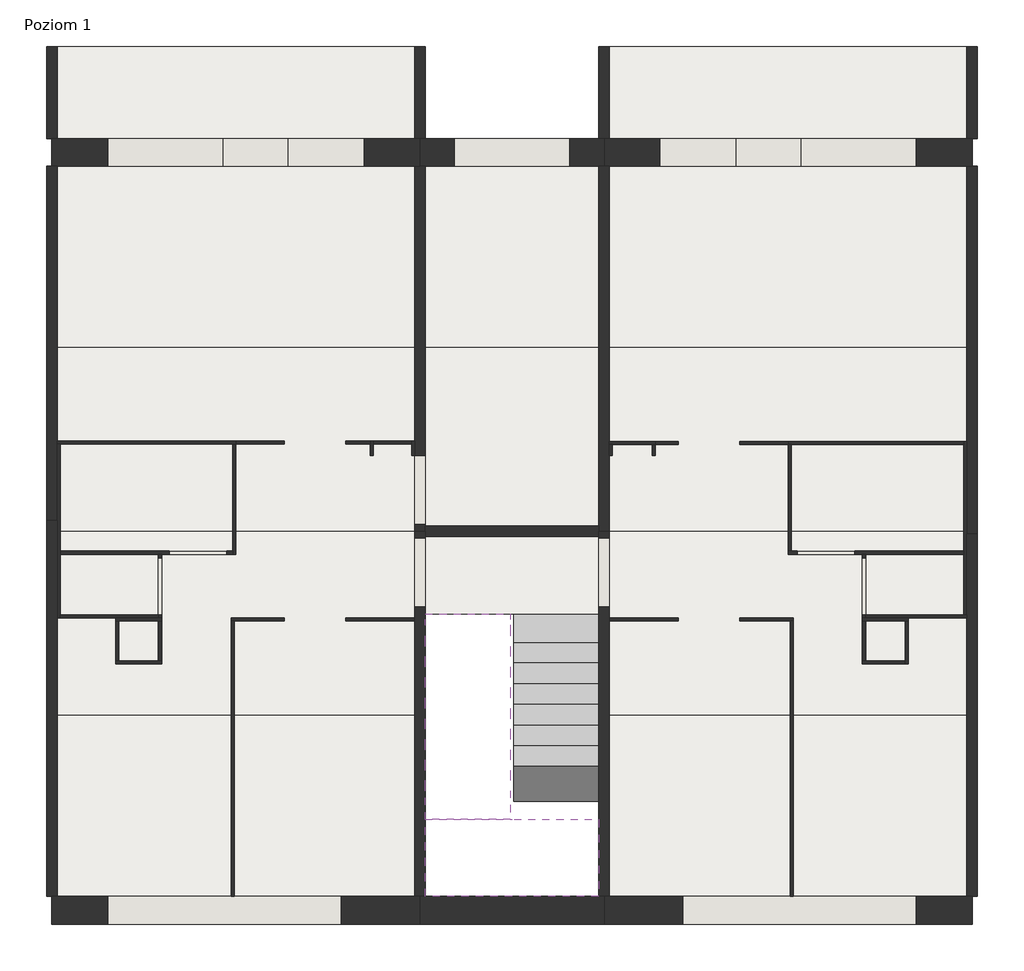
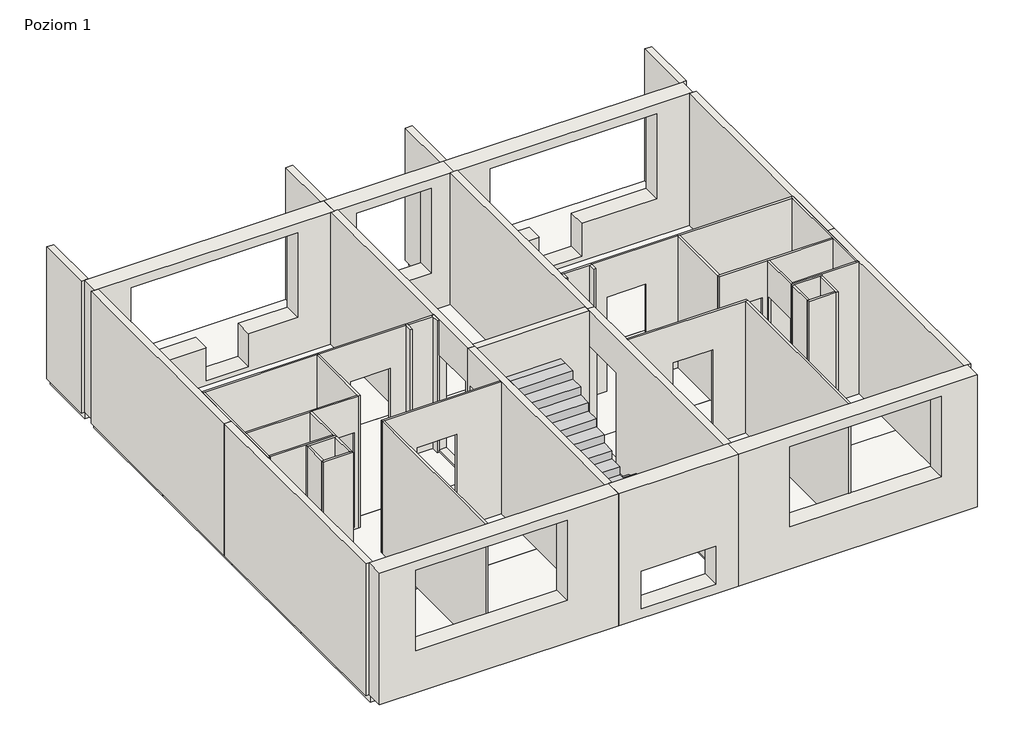
# One storey: 51 walls, 14 slabs, 2 proxies.
"""IFC4 building model written with IfcOpenShell, lengths in millimetres."""

import ifcopenshell
import ifcopenshell.guid

model = None  # the IFC model being written
_history = None  # IfcOwnerHistory: only IFC2X3 demands one
_inside = {}  # id of a spatial element -> (the spatial element, [elements in it])
_under = {}  # id of a project, library or spatial element -> (it, [spatial elements below it])
_declared = {}  # id of a project -> (the project, [libraries it declares])
_typed = {}  # id of a type object -> (the type object, [elements of that type])
_made_of = {}  # id of a material, layer set ... -> (it, [elements and type objects made of it])


def new_model(schema):
    """Start an empty IFC model of exactly this schema.

    Asked for "IFC4X3", IfcOpenShell would pick the latest addendum, in which some entities
    have other attributes; the version numbers below select the first issue.
    IFC2X3 requires an IfcOwnerHistory on every rooted entity: one is made here for all.
    """
    global model, _history
    if schema == "IFC4X3":
        model = ifcopenshell.file(schema_version=(4, 3, 0, 0))
    else:
        model = ifcopenshell.file(schema=schema)
    _inside.clear()
    _under.clear()
    _declared.clear()
    _typed.clear()
    _made_of.clear()
    _history = None
    if model.schema == "IFC2X3":
        org = make("IfcOrganization", Name="unknown")
        user = make(
            "IfcPersonAndOrganization",
            ThePerson=make("IfcPerson", FamilyName="unknown"),
            TheOrganization=org,
        )
        app = make(
            "IfcApplication",
            ApplicationDeveloper=org,
            Version="unknown",
            ApplicationFullName="unknown",
            ApplicationIdentifier="unknown",
        )
        _history = make(
            "IfcOwnerHistory",
            OwningUser=user,
            OwningApplication=app,
            ChangeAction="ADDED",
            CreationDate=0,
        )
    return model


def make(cls, **values):
    """One entity of the class cls with the attributes given. An attribute that is None is left unset."""
    return model.create_entity(
        cls, **{name: value for name, value in values.items() if value is not None}
    )


def rooted(cls, **values):
    """An entity with a GlobalId (a new one), such as an element, a storey or a relation."""
    return make(cls, GlobalId=ifcopenshell.guid.new(), OwnerHistory=_history, **values)


def si_unit(unit_type, name, prefix=None):
    """IfcSIUnit, for example si_unit("LENGTHUNIT", "METRE", prefix="MILLI")."""
    return make("IfcSIUnit", UnitType=unit_type, Prefix=prefix, Name=name)


def assignment(units):
    """IfcUnitAssignment: the units of a project."""
    return None if units is None else make("IfcUnitAssignment", Units=units)


def point(xyz):
    """IfcCartesianPoint."""
    return None if xyz is None else make("IfcCartesianPoint", Coordinates=xyz)


def direction(xyz):
    """IfcDirection."""
    return None if xyz is None else make("IfcDirection", DirectionRatios=xyz)


def frame(location, z_axis=None, x_axis=None):
    """IfcAxis2Placement3D, a coordinate frame: its origin and axes. An axis left out is left unset."""
    return make(
        "IfcAxis2Placement3D",
        Location=point(location),
        Axis=direction(z_axis),
        RefDirection=direction(x_axis),
    )


def origin():
    """The frame at (0, 0, 0) with its axes left unset."""
    return frame((0.0, 0.0, 0.0))


def origin_with_axes():
    """The frame at (0, 0, 0) with the z axis (0, 0, 1) and the x axis (1, 0, 0) written out."""
    return frame((0.0, 0.0, 0.0), z_axis=(0.0, 0.0, 1.0), x_axis=(1.0, 0.0, 0.0))


def place(relative_to, where):
    """IfcLocalPlacement: puts the frame where relative to a parent placement (None: the world)."""
    return make(
        "IfcLocalPlacement", PlacementRelTo=relative_to, RelativePlacement=where
    )


def context(
    kind, dimensions, precision=None, world=None, true_north=None, identifier=None
):
    """IfcGeometricRepresentationContext, for example the 3D "Model" context."""
    return make(
        "IfcGeometricRepresentationContext",
        ContextIdentifier=identifier,
        ContextType=kind,
        CoordinateSpaceDimension=dimensions,
        Precision=precision,
        WorldCoordinateSystem=world,
        TrueNorth=true_north,
    )


def project(units=None, contexts=None):
    """IfcProject with its units and contexts."""
    return rooted(
        "IfcProject",
        Name="project",
        RepresentationContexts=contexts,
        UnitsInContext=assignment(units),
    )


def spatial(cls, under=None, at=None, **own):
    """A site, building, storey or space (cls), placed at a placement, below another one or the project."""
    s = rooted(cls, ObjectPlacement=at, **own)
    if under is not None:
        _under.setdefault(under.id(), (under, []))[1].append(s)
    return s


def polyline(points):
    """IfcPolyline through the points."""
    return make("IfcPolyline", Points=[point(p) for p in points])


def outline(outer, holes=None, kind="AREA"):
    """IfcArbitraryClosedProfileDef: a profile drawn as a closed curve; with holes, ...WithVoids."""
    if holes is None:
        return make("IfcArbitraryClosedProfileDef", ProfileType=kind, OuterCurve=outer)
    return make(
        "IfcArbitraryProfileDefWithVoids",
        ProfileType=kind,
        OuterCurve=outer,
        InnerCurves=holes,
    )


def extrude(swept, where, along, depth):
    """IfcExtrudedAreaSolid: the profile swept, set in the frame where, extruded along a direction by depth."""
    return make(
        "IfcExtrudedAreaSolid",
        SweptArea=swept,
        Position=where,
        ExtrudedDirection=direction(along),
        Depth=depth,
    )


def faces_of(points, faces, orient=None, outer=None):
    """IfcFace entities. A face is a list of loops; a loop is a list of indices into points, from 0.

    orient and outer hold one flag for each loop. By default every Orientation is true, the
    first loop of a face is its IfcFaceOuterBound and the others are IfcFaceBound.
    """
    made = []
    for i, loops in enumerate(faces):
        bounds = []
        for j, loop in enumerate(loops):
            is_outer = j == 0 if outer is None else outer[i][j]
            bounds.append(
                make(
                    "IfcFaceOuterBound" if is_outer else "IfcFaceBound",
                    Bound=make("IfcPolyLoop", Polygon=[points[k] for k in loop]),
                    Orientation=True if orient is None else orient[i][j],
                )
            )
        made.append(make("IfcFace", Bounds=bounds))
    return made


def faceted_brep(points, faces, orient=None, outer=None, voids=None):
    """IfcFacetedBrep: a solid bounded by flat faces; with voids (closed shells), ...WithVoids."""
    shared = [point(p) for p in points]
    hull = make("IfcClosedShell", CfsFaces=faces_of(shared, faces, orient, outer))
    if voids is None:
        return make("IfcFacetedBrep", Outer=hull)
    return make(
        "IfcFacetedBrepWithVoids",
        Outer=hull,
        Voids=[
            make(cls, CfsFaces=faces_of(shared, fs, o, b)) for cls, fs, o, b in voids
        ],
    )


def shape(context_of_items, identifier, shape_type, items):
    """IfcShapeRepresentation: the items that make up one representation, for example the "Body"."""
    return make(
        "IfcShapeRepresentation",
        ContextOfItems=context_of_items,
        RepresentationIdentifier=identifier,
        RepresentationType=shape_type,
        Items=items,
    )


def source(mapping_origin, context_of_items, identifier, shape_type, items):
    """IfcRepresentationMap: a shape defined once, which mapped items show again and again."""
    return make(
        "IfcRepresentationMap",
        MappingOrigin=mapping_origin,
        MappedRepresentation=shape(context_of_items, identifier, shape_type, items),
    )


def transform(
    local_origin,
    x_axis=None,
    y_axis=None,
    z_axis=None,
    scale=None,
    scale2=None,
    scale3=None,
    uniform=True,
):
    """IfcCartesianTransformationOperator3D, or its non-uniform kind. x_axis, y_axis, z_axis: its Axis1, 2, 3."""
    if uniform:
        return make(
            "IfcCartesianTransformationOperator3D",
            Axis1=direction(x_axis),
            Axis2=direction(y_axis),
            LocalOrigin=point(local_origin),
            Scale=scale,
            Axis3=direction(z_axis),
        )
    return make(
        "IfcCartesianTransformationOperator3DnonUniform",
        Axis1=direction(x_axis),
        Axis2=direction(y_axis),
        LocalOrigin=point(local_origin),
        Scale=scale,
        Axis3=direction(z_axis),
        Scale2=scale2,
        Scale3=scale3,
    )


def mapped(mapping_source, mapping_target):
    """IfcMappedItem: shows the shape of a source again, moved by a transform."""
    return make(
        "IfcMappedItem", MappingSource=mapping_source, MappingTarget=mapping_target
    )


def made_of(thing, what):
    """Note that an element or type object is made of a material, layer set ...; save() writes the relation."""
    if what is not None:
        _made_of.setdefault(what.id(), (what, []))[1].append(thing)
    return thing


def element(
    cls,
    number,
    at=None,
    inside=None,
    cuts=None,
    type_object=None,
    material=None,
    context=None,
    identifier="Body",
    shape_type=None,
    held_by="IfcProductDefinitionShape",
    body=None,
    shapes=None,
    **own,
):
    """One element of the class cls, such as IfcWall. Its Tag is "e" and its number.

    at: its placement. inside: the storey or other place that contains it. cuts: it is an
    opening in that element (IfcRelVoidsElement). A single representation is given by context,
    identifier, shape_type and body (its items); several are given by shapes. held_by: the class
    of the entity that holds the representations. save() writes the other relations.
    """
    e = rooted(cls, Tag="e%d" % number, ObjectPlacement=at, **own)
    if body is not None:
        shapes = [shape(context, identifier, shape_type, body)]
    if shapes is not None:
        e.Representation = make(held_by, Representations=shapes)
    if inside is not None:
        _inside.setdefault(inside.id(), (inside, []))[1].append(e)
    if cuts is not None:
        rooted(
            "IfcRelVoidsElement", RelatingBuildingElement=cuts, RelatedOpeningElement=e
        )
    if type_object is not None:
        _typed.setdefault(type_object.id(), (type_object, []))[1].append(e)
    return made_of(e, material)


def aggregate(whole, parts):
    """IfcRelAggregates: a whole, such as a stair, and the parts it consists of."""
    return rooted("IfcRelAggregates", RelatingObject=whole, RelatedObjects=parts)


def save(model, path):
    """Write the relations noted so far, then the file.

    IfcRelAggregates (storeys below a building ...), IfcRelContainedInSpatialStructure (elements
    in a storey), IfcRelDefinesByType, IfcRelAssociatesMaterial and IfcRelDeclares: one each for
    every whole, place, type object, material and project.
    """
    for whole, parts in _under.values():
        aggregate(whole, parts)
    for where, things in _inside.values():
        rooted(
            "IfcRelContainedInSpatialStructure",
            RelatedElements=things,
            RelatingStructure=where,
        )
    for kind, things in _typed.values():
        rooted("IfcRelDefinesByType", RelatedObjects=things, RelatingType=kind)
    for what, things in _made_of.values():
        rooted("IfcRelAssociatesMaterial", RelatedObjects=things, RelatingMaterial=what)
    for by, libraries in _declared.values():
        rooted("IfcRelDeclares", RelatingContext=by, RelatedDefinitions=libraries)
    model.write(path)


def generic_models_1_generic_models_1_c3b3df0b(model_context):
    return source(origin(), model_context, "Body", "SweptSolid", [
        extrude(outline(polyline([(23365.484552, 1575.0), (23630.484552, 1575.0), (23630.484552, 1750.0), (23900.484552, 1750.0), (23900.484552, 1925.0), (24170.484552, 1925.0), (24170.484552, 2100.0), (24440.484552, 2100.0), (24440.484552, 2273.0), (24710.484552, 2273.0), (24710.484552, 2450.0), (24980.484552, 2450.0), (24980.484552, 2625.0), (25250.484552, 2625.0), (25250.484552, 2800.0), (25520.484552, 2800.0), (25670.484552, 2800.0), (25670.484552, 2660.0), (25525.484552, 2660.0), (23365.484552, 1260.0), (22990.484552, 1260.0), (22990.484552, 1400.0), (23365.484552, 1400.0), (23365.484552, 1575.0)])), frame((81451.2978475, 0.0, 0.0), z_axis=(1.0, 0.0, 0.0), x_axis=(0.0, 1.0, 0.0)), (0.0, 0.0, 1.0), 1105.7161874),
    ])


def generic_models_3_generic_models_1_35d45e08(model_context):
    return source(origin(), model_context, "Body", "SweptSolid", [
        extrude(outline(polyline([(25295.484552, 175.0), (25295.484552, 0.0), (25670.484552, 0.0), (25670.484552, -140.0), (25295.484552, -140.0), (23135.484552, 1260.0), (22990.484552, 1260.0), (22990.484552, 1400.0), (23140.484552, 1400.0), (23410.484552, 1400.0), (23410.484552, 1225.0), (23680.484552, 1225.0), (23680.484552, 1050.0), (23950.484552, 1050.0), (23950.484552, 873.0), (24220.484552, 873.0), (24220.484552, 700.0), (24490.484552, 700.0), (24490.484552, 525.0), (24760.484552, 525.0), (24760.484552, 350.0), (25030.484552, 350.0), (25030.484552, 175.0), (25295.484552, 175.0)])), frame((82605.5816601, 0.0, 0.0), z_axis=(1.0, 0.0, 0.0), x_axis=(0.0, 1.0, 0.0)), (0.0, 0.0, 1.0), 1105.7161874),
    ])


model = new_model("IFC4")

# Units and contexts
model_context = context("Model", 3, world=origin())
ifc_project = project(units=[si_unit("LENGTHUNIT", "METRE", prefix="MILLI")], contexts=[model_context])

# Site, building, storey
site = spatial("IfcSite", under=ifc_project)
building = spatial("IfcBuilding", under=site)
storey = spatial("IfcBuildingStorey", under=building, Name="Poziom 1", Elevation=0.0)

# Proxies
placement = place(None, origin())
generic_models_1_generic_models_1_shape = generic_models_1_generic_models_1_c3b3df0b(model_context)
element("IfcBuildingElementProxy", 1, Name="Generic Models 1 : Generic Models 1", ObjectType="Generic Models 1 : Generic Models 1", at=placement, inside=storey, context=model_context, shape_type="MappedRepresentation", body=[
    mapped(generic_models_1_generic_models_1_shape, transform((0.0, 0.0, 0.0), x_axis=(1.0, 0.0, 0.0), y_axis=(0.0, 1.0, 0.0), z_axis=(0.0, 0.0, 1.0))),
])
generic_models_3_generic_models_1_shape = generic_models_3_generic_models_1_35d45e08(model_context)
element("IfcBuildingElementProxy", 2, Name="Generic Models 3 : Generic Models 1", ObjectType="Generic Models 3 : Generic Models 1", at=placement, inside=storey, context=model_context, shape_type="MappedRepresentation", body=[
    mapped(generic_models_3_generic_models_1_shape, transform((0.0, 0.0, 0.0), x_axis=(1.0, 0.0, 0.0), y_axis=(0.0, 1.0, 0.0), z_axis=(0.0, 0.0, 1.0))),
])

# Slabs
element("IfcSlab", 3, ObjectType="Prefab_slab", at=placement, inside=storey, context=model_context, shape_type="SweptSolid", body=[
    extrude(outline(polyline([(81381.2978475, 24350.484552), (81381.2978475, 21950.484552), (76581.2978475, 21950.484552), (76581.2978475, 24350.484552), (81381.2978475, 24350.484552)])), frame((0.0, 0.0, -140.0), z_axis=(0.0, 0.0, 1.0), x_axis=(1.0, 0.0, 0.0)), (0.0, 0.0, 1.0), 140.0),
])
element("IfcSlab", 4, ObjectType="Prefab_slab", at=placement, inside=storey, context=model_context, shape_type="SweptSolid", body=[
    extrude(outline(polyline([(81381.2978475, 26750.484552), (81381.2978475, 24350.484552), (76581.2978475, 24350.484552), (76581.2978475, 26750.484552), (81381.2978475, 26750.484552)])), frame((0.0, 0.0, -140.0), z_axis=(0.0, 0.0, 1.0), x_axis=(1.0, 0.0, 0.0)), (0.0, 0.0, 1.0), 140.0),
])
element("IfcSlab", 5, ObjectType="Prefab_slab", at=placement, inside=storey, context=model_context, shape_type="SweptSolid", body=[
    extrude(outline(polyline([(81381.2978475, 29150.484552), (81381.2978475, 26750.484552), (76581.2978475, 26750.484552), (76581.2978475, 29150.484552), (81381.2978475, 29150.484552)])), frame((0.0, 0.0, -140.0), z_axis=(0.0, 0.0, 1.0), x_axis=(1.0, 0.0, 0.0)), (0.0, 0.0, 1.0), 140.0),
])
element("IfcSlab", 6, ObjectType="Prefab_slab", at=placement, inside=storey, context=model_context, shape_type="SweptSolid", body=[
    extrude(outline(polyline([(81381.2978475, 31550.484552), (81381.2978475, 29150.484552), (76581.2978475, 29150.484552), (76581.2978475, 31550.484552), (81381.2978475, 31550.484552)])), frame((0.0, 0.0, -140.0), z_axis=(0.0, 0.0, 1.0), x_axis=(1.0, 0.0, 0.0)), (0.0, 0.0, 1.0), 140.0),
])
element("IfcSlab", 7, ObjectType="Prefab_slab", at=placement, inside=storey, context=model_context, shape_type="SweptSolid", body=[
    extrude(outline(polyline([(88581.2978475, 24350.484552), (88581.2978475, 21950.484552), (83781.2978475, 21950.484552), (83781.2978475, 24350.484552), (88581.2978475, 24350.484552)])), frame((0.0, 0.0, -140.0), z_axis=(0.0, 0.0, 1.0), x_axis=(1.0, 0.0, 0.0)), (0.0, 0.0, 1.0), 140.0),
])
element("IfcSlab", 8, ObjectType="Prefab_slab", at=placement, inside=storey, context=model_context, shape_type="SweptSolid", body=[
    extrude(outline(polyline([(88581.2978475, 26750.484552), (88581.2978475, 24350.484552), (83781.2978475, 24350.484552), (83781.2978475, 26750.484552), (88581.2978475, 26750.484552)])), frame((0.0, 0.0, -140.0), z_axis=(0.0, 0.0, 1.0), x_axis=(1.0, 0.0, 0.0)), (0.0, 0.0, 1.0), 140.0),
])
element("IfcSlab", 9, ObjectType="Prefab_slab", at=placement, inside=storey, context=model_context, shape_type="SweptSolid", body=[
    extrude(outline(polyline([(88581.2978475, 29150.484552), (88581.2978475, 26750.484552), (83781.2978475, 26750.484552), (83781.2978475, 29150.484552), (88581.2978475, 29150.484552)])), frame((0.0, 0.0, -140.0), z_axis=(0.0, 0.0, 1.0), x_axis=(1.0, 0.0, 0.0)), (0.0, 0.0, 1.0), 140.0),
])
element("IfcSlab", 10, ObjectType="Prefab_slab", at=placement, inside=storey, context=model_context, shape_type="SweptSolid", body=[
    extrude(outline(polyline([(88581.2978475, 31550.484552), (88581.2978475, 29150.484552), (83781.2978475, 29150.484552), (83781.2978475, 31550.484552), (88581.2978475, 31550.484552)])), frame((0.0, 0.0, -140.0), z_axis=(0.0, 0.0, 1.0), x_axis=(1.0, 0.0, 0.0)), (0.0, 0.0, 1.0), 140.0),
])
element("IfcSlab", 11, ObjectType="Prefab_slab", at=placement, inside=storey, context=model_context, shape_type="SweptSolid", body=[
    extrude(outline(polyline([(83781.2978475, 31550.484552), (83781.2978475, 29150.484552), (81451.2978475, 29150.484552), (81451.2978475, 31550.484552), (83781.2978475, 31550.484552)])), frame((0.0, 0.0, -140.0), z_axis=(0.0, 0.0, 1.0), x_axis=(1.0, 0.0, 0.0)), (0.0, 0.0, 1.0), 140.0),
])
element("IfcSlab", 12, ObjectType="Prefab_slab", at=placement, inside=storey, context=model_context, shape_type="SweptSolid", body=[
    extrude(outline(polyline([(83781.2978475, 29150.484552), (83781.2978475, 26750.484552), (81451.2978475, 26750.484552), (81451.2978475, 29150.484552), (83781.2978475, 29150.484552)])), frame((0.0, 0.0, -140.0), z_axis=(0.0, 0.0, 1.0), x_axis=(1.0, 0.0, 0.0)), (0.0, 0.0, 1.0), 140.0),
])
element("IfcSlab", 13, ObjectType="Prefab_slab", at=placement, inside=storey, context=model_context, shape_type="SweptSolid", body=[
    extrude(outline(polyline([(83781.2978475, 26750.484552), (83781.2978475, 25670.484552), (81451.2978475, 25670.484552), (81451.2978475, 26750.484552), (83781.2978475, 26750.484552)])), frame((0.0, 0.0, -140.0), z_axis=(0.0, 0.0, 1.0), x_axis=(1.0, 0.0, 0.0)), (0.0, 0.0, 1.0), 140.0),
])
element("IfcSlab", 14, ObjectType="Prefab_slab", at=placement, inside=storey, context=model_context, shape_type="SweptSolid", body=[
    extrude(outline(polyline([(83711.2978475, 22990.484552), (83711.2978475, 21985.484552), (81451.2978475, 21985.484552), (81451.2978475, 22990.484552), (82558.3014634, 22990.484552), (82611.2978475, 22990.484552), (83711.2978475, 22990.484552)])), frame((0.0, 0.0, 1260.0), z_axis=(0.0, 0.0, 1.0), x_axis=(1.0, 0.0, 0.0)), (0.0, 0.0, 1.0), 140.0),
])
element("IfcSlab", 15, ObjectType="Prefab_slab 2", at=placement, inside=storey, context=model_context, shape_type="SweptSolid", body=[
    extrude(outline(polyline([(81381.2978475, 33075.484552), (81381.2978475, 31875.484552), (76581.2978475, 31875.484552), (76581.2978475, 33075.484552), (81381.2978475, 33075.484552)])), frame((0.0, 0.0, -140.0), z_axis=(0.0, 0.0, 1.0), x_axis=(1.0, 0.0, 0.0)), (0.0, 0.0, 1.0), 140.0),
])
element("IfcSlab", 16, ObjectType="Prefab_slab 2", at=placement, inside=storey, context=model_context, shape_type="SweptSolid", body=[
    extrude(outline(polyline([(88581.2978475, 33075.484552), (88581.2978475, 31875.484552), (83781.2978475, 31875.484552), (83781.2978475, 33075.484552), (88581.2978475, 33075.484552)])), frame((0.0, 0.0, -140.0), z_axis=(0.0, 0.0, 1.0), x_axis=(1.0, 0.0, 0.0)), (0.0, 0.0, 1.0), 140.0),
])

# Walls
element("IfcWall", 17, ObjectType="Prefab_ext_wall", at=placement, inside=storey, context=model_context, shape_type="SweptSolid", body=[
    extrude(outline(polyline([(0.0, 76581.2978475), (0.0, 81381.2978475), (2800.0, 81381.2978475), (2800.0, 76581.2978475), (0.0, 76581.2978475)]), holes=[polyline([(2600.0, 77311.2978475), (2600.0, 80651.2978475), (800.0, 80651.2978475), (800.0, 79661.2978475), (100.0, 79661.2978475), (100.0, 78811.2978475), (800.0, 78811.2978475), (800.0, 77311.2978475), (2600.0, 77311.2978475)])]), frame((0.0, 31515.484552, 0.0), z_axis=(0.0, 1.0, 0.0), x_axis=(0.0, 0.0, 1.0)), (0.0, 0.0, 1.0), 360.0),
])
element("IfcWall", 18, ObjectType="Prefab_ext_wall", at=placement, inside=storey, context=model_context, shape_type="SweptSolid", body=[
    extrude(outline(polyline([(0.0, 81381.2978475), (0.0, 83781.2978475), (2800.0, 83781.2978475), (2800.0, 81381.2978475), (0.0, 81381.2978475)]), holes=[polyline([(800.0, 83331.2978475), (800.0, 81831.2978475), (2600.0, 81831.2978475), (2600.0, 83331.2978475), (800.0, 83331.2978475)])]), frame((0.0, 31515.484552, 0.0), z_axis=(0.0, 1.0, 0.0), x_axis=(0.0, 0.0, 1.0)), (0.0, 0.0, 1.0), 360.0),
])
element("IfcWall", 19, ObjectType="Prefab_ext_wall", at=placement, inside=storey, context=model_context, shape_type="SweptSolid", body=[
    extrude(outline(polyline([(0.0, 83781.2978475), (0.0, 88581.2978475), (2800.0, 88581.2978475), (2800.0, 83781.2978475), (0.0, 83781.2978475)]), holes=[polyline([(800.0, 84511.2978475), (2600.0, 84511.2978475), (2600.0, 87851.2978475), (800.0, 87851.2978475), (800.0, 86351.2978475), (100.0, 86351.2978475), (100.0, 85501.2978475), (800.0, 85501.2978475), (800.0, 84511.2978475)])]), frame((0.0, 31515.484552, 0.0), z_axis=(0.0, 1.0, 0.0), x_axis=(0.0, 0.0, 1.0)), (0.0, 0.0, 1.0), 360.0),
])
element("IfcWall", 20, ObjectType="Prefab_ext_wall", at=placement, inside=storey, context=model_context, shape_type="SweptSolid", body=[
    extrude(outline(polyline([(0.0, 76581.2978475), (0.0, 81381.2978475), (2800.0, 81381.2978475), (2800.0, 76581.2978475), (0.0, 76581.2978475)]), holes=[polyline([(2600.0, 77311.2978475), (2600.0, 80351.2978475), (900.0, 80351.2978475), (900.0, 77311.2978475), (2600.0, 77311.2978475)])]), frame((0.0, 21625.484552, 0.0), z_axis=(0.0, 1.0, 0.0), x_axis=(0.0, 0.0, 1.0)), (0.0, 0.0, 1.0), 360.0),
])
element("IfcWall", 21, ObjectType="Prefab_ext_wall", at=placement, inside=storey, context=model_context, shape_type="SweptSolid", body=[
    extrude(outline(polyline([(0.0, 81381.2978475), (0.0, 83781.2978475), (2800.0, 83781.2978475), (2800.0, 81381.2978475), (0.0, 81381.2978475)]), holes=[polyline([(1000.0, 83331.2978475), (200.0, 83331.2978475), (200.0, 81831.2978475), (1000.0, 81831.2978475), (1000.0, 83331.2978475)])]), frame((0.0, 21625.484552, 0.0), z_axis=(0.0, 1.0, 0.0), x_axis=(0.0, 0.0, 1.0)), (0.0, 0.0, 1.0), 360.0),
])
element("IfcWall", 22, ObjectType="Prefab_ext_wall", at=placement, inside=storey, context=model_context, shape_type="SweptSolid", body=[
    extrude(outline(polyline([(0.0, 83781.2978475), (0.0, 88581.2978475), (2800.0, 88581.2978475), (2800.0, 83781.2978475), (0.0, 83781.2978475)]), holes=[polyline([(900.0, 87851.2978475), (900.0, 84811.2978475), (2600.0, 84811.2978475), (2600.0, 87851.2978475), (900.0, 87851.2978475)])]), frame((0.0, 21625.484552, 0.0), z_axis=(0.0, 1.0, 0.0), x_axis=(0.0, 0.0, 1.0)), (0.0, 0.0, 1.0), 360.0),
])
element("IfcWall", 23, ObjectType="Prefab_int_wall", at=placement, inside=storey, context=model_context, shape_type="Brep", body=[
    faceted_brep([(76651.2978475, 27890.484552, 0.0), (76691.2978475, 27890.484552, 0.0), (78941.2978475, 27890.484552, 0.0), (78981.2978475, 27890.484552, 0.0), (78981.2978475, 27890.484552, 2800.0), (78941.2978475, 27890.484552, 2800.0), (76691.2978475, 27890.484552, 2800.0), (76651.2978475, 27890.484552, 2800.0), (76651.2978475, 27930.484552, 0.0), (76651.2978475, 27930.484552, 2800.0), (78981.2978475, 27930.484552, 2800.0), (78981.2978475, 27930.484552, 0.0)], [[[0, 1, 2, 3, 4, 5, 6, 7]], [[8, 9, 10, 11]], [[3, 2, 1, 0, 8, 11]], [[4, 3, 11, 10]], [[7, 6, 5, 4, 10, 9]], [[0, 7, 9, 8]]]),
])
element("IfcWall", 24, ObjectType="Prefab_int_wall", at=placement, inside=storey, context=model_context, shape_type="Brep", body=[
    faceted_brep([(78921.2978475, 25580.484552, 0.0), (78961.2978475, 25580.484552, 0.0), (79611.2978475, 25580.484552, 0.0), (79611.2978475, 25580.484552, 2000.0), (80411.2978475, 25580.484552, 2000.0), (80411.2978475, 25580.484552, 0.0), (81311.2978475, 25580.484552, 0.0), (81311.2978475, 25580.484552, 2800.0), (78961.2978475, 25580.484552, 2800.0), (78921.2978475, 25580.484552, 2800.0), (78921.2978475, 25620.484552, 0.0), (78921.2978475, 25620.484552, 2800.0), (81311.2978475, 25620.484552, 2800.0), (81311.2978475, 25620.484552, 0.0), (80411.2978475, 25620.484552, 0.0), (80411.2978475, 25620.484552, 2000.0), (79611.2978475, 25620.484552, 2000.0), (79611.2978475, 25620.484552, 0.0)], [[[0, 1, 2, 3, 4, 5, 6, 7, 8, 9]], [[10, 11, 12, 13, 14, 15, 16, 17]], [[6, 5, 14, 13]], [[7, 6, 13, 12]], [[9, 8, 7, 12, 11]], [[2, 1, 0, 10, 17]], [[3, 2, 17, 16]], [[4, 3, 16, 15]], [[5, 4, 15, 14]], [[0, 9, 11, 10]]]),
])
element("IfcWall", 25, ObjectType="Prefab_int_wall", at=placement, inside=storey, context=model_context, shape_type="SweptSolid", body=[
    extrude(outline(polyline([(78921.2978475, 21985.484552), (78921.2978475, 25580.484552), (78961.2978475, 25580.484552), (78961.2978475, 21985.484552), (78921.2978475, 21985.484552)])), origin_with_axes(), (0.0, 0.0, 1.0), 2800.0),
])
element("IfcWall", 26, ObjectType="Prefab_int_wall", at=placement, inside=storey, context=model_context, shape_type="Brep", body=[
    faceted_brep([(83851.2978475, 25580.484552, 0.0), (84751.2978475, 25580.484552, 0.0), (84751.2978475, 25580.484552, 2000.0), (85551.2978475, 25580.484552, 2000.0), (85551.2978475, 25580.484552, 0.0), (86211.2978475, 25580.484552, 0.0), (86251.2978475, 25580.484552, 0.0), (86251.2978475, 25580.484552, 2800.0), (86211.2978475, 25580.484552, 2800.0), (83851.2978475, 25580.484552, 2800.0), (83851.2978475, 25620.484552, 0.0), (83851.2978475, 25620.484552, 2800.0), (86251.2978475, 25620.484552, 2800.0), (86251.2978475, 25620.484552, 0.0), (85551.2978475, 25620.484552, 0.0), (85551.2978475, 25620.484552, 2000.0), (84751.2978475, 25620.484552, 2000.0), (84751.2978475, 25620.484552, 0.0)], [[[0, 1, 2, 3, 4, 5, 6, 7, 8, 9]], [[10, 11, 12, 13, 14, 15, 16, 17]], [[7, 6, 13, 12]], [[0, 9, 11, 10]], [[6, 5, 4, 14, 13]], [[9, 8, 7, 12, 11]], [[1, 0, 10, 17]], [[2, 1, 17, 16]], [[3, 2, 16, 15]], [[4, 3, 15, 14]]]),
])
element("IfcWall", 27, ObjectType="Prefab_int_wall", at=placement, inside=storey, context=model_context, shape_type="SweptSolid", body=[
    extrude(outline(polyline([(86211.2978475, 21985.484552), (86211.2978475, 25580.484552), (86251.2978475, 25580.484552), (86251.2978475, 21985.484552), (86211.2978475, 21985.484552)])), origin_with_axes(), (0.0, 0.0, 1.0), 2800.0),
])
element("IfcWall", 28, ObjectType="Prefab_int_wall", at=placement, inside=storey, context=model_context, shape_type="Brep", body=[
    faceted_brep([(87151.2978475, 25580.484552, 0.0), (87191.2978475, 25580.484552, 0.0), (87711.2978475, 25580.484552, 0.0), (87751.2978475, 25580.484552, 0.0), (87751.2978475, 25580.484552, 2800.0), (87711.2978475, 25580.484552, 2800.0), (87191.2978475, 25580.484552, 2800.0), (87151.2978475, 25580.484552, 2800.0), (87151.2978475, 25620.484552, 0.0), (87151.2978475, 25620.484552, 2800.0), (87751.2978475, 25620.484552, 2800.0), (87751.2978475, 25620.484552, 0.0)], [[[0, 1, 2, 3, 4, 5, 6, 7]], [[8, 9, 10, 11]], [[3, 2, 1, 0, 8, 11]], [[7, 6, 5, 4, 10, 9]], [[4, 3, 11, 10]], [[0, 7, 9, 8]]]),
])
element("IfcWall", 29, ObjectType="Prefab_int_wall", at=placement, inside=storey, context=model_context, shape_type="Brep", body=[
    faceted_brep([(87711.2978475, 25580.484552, 0.0), (87711.2978475, 25060.484552, 0.0), (87711.2978475, 25020.484552, 0.0), (87711.2978475, 25020.484552, 2800.0), (87711.2978475, 25060.484552, 2800.0), (87711.2978475, 25580.484552, 2800.0), (87751.2978475, 25580.484552, 0.0), (87751.2978475, 25580.484552, 2800.0), (87751.2978475, 25020.484552, 2800.0), (87751.2978475, 25020.484552, 0.0)], [[[0, 1, 2, 3, 4, 5]], [[6, 7, 8, 9]], [[2, 1, 0, 6, 9]], [[5, 4, 3, 8, 7]], [[0, 5, 7, 6]], [[3, 2, 9, 8]]]),
])
element("IfcWall", 30, ObjectType="Prefab_int_wall", at=placement, inside=storey, context=model_context, shape_type="Brep", body=[
    faceted_brep([(87711.2978475, 25060.484552, 0.0), (87191.2978475, 25060.484552, 0.0), (87151.2978475, 25060.484552, 0.0), (87151.2978475, 25060.484552, 2800.0), (87191.2978475, 25060.484552, 2800.0), (87711.2978475, 25060.484552, 2800.0), (87711.2978475, 25020.484552, 0.0), (87711.2978475, 25020.484552, 2800.0), (87151.2978475, 25020.484552, 2800.0), (87151.2978475, 25020.484552, 0.0)], [[[0, 1, 2, 3, 4, 5]], [[6, 7, 8, 9]], [[2, 1, 0, 6, 9]], [[5, 4, 3, 8, 7]], [[0, 5, 7, 6]], [[3, 2, 9, 8]]]),
])
element("IfcWall", 31, ObjectType="Prefab_int_wall", at=placement, inside=storey, context=model_context, shape_type="Brep", body=[
    faceted_brep([(87191.2978475, 25620.484552, 0.0), (87191.2978475, 25660.484552, 0.0), (87191.2978475, 26450.484552, 0.0), (87191.2978475, 26450.484552, 2800.0), (87191.2978475, 25660.484552, 2800.0), (87191.2978475, 25620.484552, 2800.0), (87191.2978475, 26400.484552, 2050.0), (87191.2978475, 26400.484552, 50.0), (87191.2978475, 25660.484552, 50.0), (87191.2978475, 25660.484552, 2050.0), (87151.2978475, 25620.484552, 0.0), (87151.2978475, 25620.484552, 2800.0), (87151.2978475, 26450.484552, 2800.0), (87151.2978475, 26450.484552, 0.0), (87151.2978475, 26400.484552, 2050.0), (87151.2978475, 25660.484552, 2050.0), (87151.2978475, 25660.484552, 50.0), (87151.2978475, 26400.484552, 50.0)], [[[0, 1, 2, 3, 4, 5], [6, 7, 8, 9]], [[10, 11, 12, 13], [14, 15, 16, 17]], [[3, 2, 13, 12]], [[2, 1, 0, 10, 13]], [[5, 4, 3, 12, 11]], [[0, 5, 11, 10]], [[7, 6, 14, 17]], [[8, 7, 17, 16]], [[6, 9, 15, 14]], [[9, 8, 16, 15]]]),
])
element("IfcWall", 32, ObjectType="Prefab_int_wall", at=placement, inside=storey, context=model_context, shape_type="Brep", body=[
    faceted_brep([(77411.2978475, 25580.484552, 0.0), (77451.2978475, 25580.484552, 0.0), (77971.2978475, 25580.484552, 0.0), (78011.2978475, 25580.484552, 0.0), (78011.2978475, 25580.484552, 2800.0), (77971.2978475, 25580.484552, 2800.0), (77451.2978475, 25580.484552, 2800.0), (77411.2978475, 25580.484552, 2800.0), (77411.2978475, 25620.484552, 0.0), (77411.2978475, 25620.484552, 2800.0), (78011.2978475, 25620.484552, 2800.0), (78011.2978475, 25620.484552, 0.0)], [[[0, 1, 2, 3, 4, 5, 6, 7]], [[8, 9, 10, 11]], [[3, 2, 1, 0, 8, 11]], [[7, 6, 5, 4, 10, 9]], [[0, 7, 9, 8]], [[4, 3, 11, 10]]]),
])
element("IfcWall", 33, ObjectType="Prefab_int_wall", at=placement, inside=storey, context=model_context, shape_type="Brep", body=[
    faceted_brep([(77971.2978475, 26450.484552, 0.0), (77971.2978475, 25660.484552, 0.0), (77971.2978475, 25620.484552, 0.0), (77971.2978475, 25620.484552, 2800.0), (77971.2978475, 25660.484552, 2800.0), (77971.2978475, 26450.484552, 2800.0), (77971.2978475, 25660.484552, 50.0), (77971.2978475, 26400.484552, 50.0), (77971.2978475, 26400.484552, 2050.0), (77971.2978475, 25660.484552, 2050.0), (78011.2978475, 26450.484552, 0.0), (78011.2978475, 26450.484552, 2800.0), (78011.2978475, 25620.484552, 2800.0), (78011.2978475, 25620.484552, 0.0), (78011.2978475, 25660.484552, 50.0), (78011.2978475, 25660.484552, 2050.0), (78011.2978475, 26400.484552, 2050.0), (78011.2978475, 26400.484552, 50.0)], [[[0, 1, 2, 3, 4, 5], [6, 7, 8, 9]], [[10, 11, 12, 13], [14, 15, 16, 17]], [[0, 5, 11, 10]], [[2, 1, 0, 10, 13]], [[3, 2, 13, 12]], [[5, 4, 3, 12, 11]], [[7, 6, 14, 17]], [[8, 7, 17, 16]], [[9, 8, 16, 15]], [[6, 9, 15, 14]]]),
])
element("IfcWall", 34, ObjectType="Prefab_int_wall", at=placement, inside=storey, context=model_context, shape_type="Brep", body=[
    faceted_brep([(78011.2978475, 25060.484552, 0.0), (77971.2978475, 25060.484552, 0.0), (77451.2978475, 25060.484552, 0.0), (77411.2978475, 25060.484552, 0.0), (77411.2978475, 25060.484552, 2800.0), (77451.2978475, 25060.484552, 2800.0), (77971.2978475, 25060.484552, 2800.0), (78011.2978475, 25060.484552, 2800.0), (78011.2978475, 25020.484552, 0.0), (78011.2978475, 25020.484552, 2800.0), (77411.2978475, 25020.484552, 2800.0), (77411.2978475, 25020.484552, 0.0)], [[[0, 1, 2, 3, 4, 5, 6, 7]], [[8, 9, 10, 11]], [[3, 2, 1, 0, 8, 11]], [[7, 6, 5, 4, 10, 9]], [[4, 3, 11, 10]], [[0, 7, 9, 8]]]),
])
element("IfcWall", 35, ObjectType="Prefab_int_wall", at=placement, inside=storey, context=model_context, shape_type="SweptSolid", body=[
    extrude(outline(polyline([(77451.2978475, 25580.484552), (77451.2978475, 25060.484552), (77411.2978475, 25060.484552), (77411.2978475, 25580.484552), (77451.2978475, 25580.484552)])), origin_with_axes(), (0.0, 0.0, 1.0), 2800.0),
])
element("IfcWall", 36, ObjectType="Prefab_int_wall", at=placement, inside=storey, context=model_context, shape_type="Brep", body=[
    faceted_brep([(78941.2978475, 27890.484552, 0.0), (78941.2978475, 26490.484552, 0.0), (78941.2978475, 26450.484552, 0.0), (78941.2978475, 26450.484552, 2800.0), (78941.2978475, 26490.484552, 2800.0), (78941.2978475, 27890.484552, 2800.0), (78981.2978475, 27890.484552, 0.0), (78981.2978475, 27890.484552, 2800.0), (78981.2978475, 26450.484552, 2800.0), (78981.2978475, 26450.484552, 0.0)], [[[0, 1, 2, 3, 4, 5]], [[6, 7, 8, 9]], [[2, 1, 0, 6, 9]], [[5, 4, 3, 8, 7]], [[3, 2, 9, 8]], [[0, 5, 7, 6]]]),
])
element("IfcWall", 37, ObjectType="Prefab_int_wall", at=placement, inside=storey, context=model_context, shape_type="Brep", body=[
    faceted_brep([(78941.2978475, 26490.484552, 0.0), (76691.2978475, 26490.484552, 0.0), (76691.2978475, 26490.484552, 2800.0), (78941.2978475, 26490.484552, 2800.0), (78111.2978475, 26490.484552, 50.0), (78861.2978475, 26490.484552, 50.0), (78861.2978475, 26490.484552, 2050.0), (78111.2978475, 26490.484552, 2050.0), (78941.2978475, 26450.484552, 0.0), (78941.2978475, 26450.484552, 2800.0), (78011.2978475, 26450.484552, 2800.0), (77971.2978475, 26450.484552, 2800.0), (76691.2978475, 26450.484552, 2800.0), (76691.2978475, 26450.484552, 0.0), (77971.2978475, 26450.484552, 0.0), (78011.2978475, 26450.484552, 0.0), (78111.2978475, 26450.484552, 50.0), (78111.2978475, 26450.484552, 2050.0), (78861.2978475, 26450.484552, 2050.0), (78861.2978475, 26450.484552, 50.0)], [[[0, 1, 2, 3], [4, 5, 6, 7]], [[8, 9, 10, 11, 12, 13, 14, 15], [16, 17, 18, 19]], [[0, 3, 9, 8]], [[2, 1, 13, 12]], [[1, 0, 8, 15, 14, 13]], [[3, 2, 12, 11, 10, 9]], [[5, 4, 16, 19]], [[6, 5, 19, 18]], [[7, 6, 18, 17]], [[4, 7, 17, 16]]]),
])
element("IfcWall", 38, ObjectType="Prefab_int_wall", at=placement, inside=storey, context=model_context, shape_type="Brep", body=[
    faceted_brep([(76691.2978475, 25620.484552, 0.0), (76691.2978475, 25660.484552, 0.0), (76691.2978475, 26450.484552, 0.0), (76691.2978475, 26490.484552, 0.0), (76691.2978475, 27890.484552, 0.0), (76691.2978475, 27890.484552, 2800.0), (76691.2978475, 26490.484552, 2800.0), (76691.2978475, 26450.484552, 2800.0), (76691.2978475, 25660.484552, 2800.0), (76691.2978475, 25620.484552, 2800.0), (76651.2978475, 25620.484552, 0.0), (76651.2978475, 25620.484552, 2800.0), (76651.2978475, 27890.484552, 2800.0), (76651.2978475, 27890.484552, 0.0)], [[[0, 1, 2, 3, 4, 5, 6, 7, 8, 9]], [[10, 11, 12, 13]], [[4, 3, 2, 1, 0, 10, 13]], [[9, 8, 7, 6, 5, 12, 11]], [[0, 9, 11, 10]], [[5, 4, 13, 12]]]),
])
element("IfcWall", 39, ObjectType="Prefab_int_wall", at=placement, inside=storey, context=model_context, shape_type="Brep", body=[
    faceted_brep([(88511.2978475, 25660.484552, 0.0), (88471.2978475, 25660.484552, 0.0), (87191.2978475, 25660.484552, 0.0), (87191.2978475, 25660.484552, 50.0), (87191.2978475, 25660.484552, 2050.0), (87191.2978475, 25660.484552, 2800.0), (88471.2978475, 25660.484552, 2800.0), (88511.2978475, 25660.484552, 2800.0), (88511.2978475, 25620.484552, 0.0), (88511.2978475, 25620.484552, 2800.0), (87191.2978475, 25620.484552, 2800.0), (87191.2978475, 25620.484552, 0.0)], [[[0, 1, 2, 3, 4, 5, 6, 7]], [[8, 9, 10, 11]], [[2, 1, 0, 8, 11]], [[7, 6, 5, 10, 9]], [[0, 7, 9, 8]], [[2, 11, 10, 5, 4, 3]]]),
])
element("IfcWall", 40, ObjectType="Prefab_int_wall", at=placement, inside=storey, context=model_context, shape_type="Brep", body=[
    faceted_brep([(88471.2978475, 26490.484552, 0.0), (86221.2978475, 26490.484552, 0.0), (86181.2978475, 26490.484552, 0.0), (86181.2978475, 26490.484552, 2800.0), (86221.2978475, 26490.484552, 2800.0), (88471.2978475, 26490.484552, 2800.0), (86301.2978475, 26490.484552, 2050.0), (86301.2978475, 26490.484552, 50.0), (87051.2978475, 26490.484552, 50.0), (87051.2978475, 26490.484552, 2050.0), (88471.2978475, 26450.484552, 0.0), (88471.2978475, 26450.484552, 2800.0), (87191.2978475, 26450.484552, 2800.0), (87151.2978475, 26450.484552, 2800.0), (86181.2978475, 26450.484552, 2800.0), (86181.2978475, 26450.484552, 0.0), (87151.2978475, 26450.484552, 0.0), (87191.2978475, 26450.484552, 0.0), (86301.2978475, 26450.484552, 2050.0), (87051.2978475, 26450.484552, 2050.0), (87051.2978475, 26450.484552, 50.0), (86301.2978475, 26450.484552, 50.0)], [[[0, 1, 2, 3, 4, 5], [6, 7, 8, 9]], [[10, 11, 12, 13, 14, 15, 16, 17], [18, 19, 20, 21]], [[3, 2, 15, 14]], [[0, 5, 11, 10]], [[2, 1, 0, 10, 17, 16, 15]], [[5, 4, 3, 14, 13, 12, 11]], [[7, 6, 18, 21]], [[8, 7, 21, 20]], [[9, 8, 20, 19]], [[6, 9, 19, 18]]]),
])
element("IfcWall", 41, ObjectType="Prefab_int_wall", at=placement, inside=storey, context=model_context, shape_type="SweptSolid", body=[
    extrude(outline(polyline([(86221.2978475, 27880.484552), (86221.2978475, 26490.484552), (86181.2978475, 26490.484552), (86181.2978475, 27880.484552), (86221.2978475, 27880.484552)])), origin_with_axes(), (0.0, 0.0, 1.0), 2800.0),
])
element("IfcWall", 42, ObjectType="Prefab_int_wall", at=placement, inside=storey, context=model_context, shape_type="Brep", body=[
    faceted_brep([(88471.2978475, 27920.484552, 0.0), (88471.2978475, 27880.484552, 0.0), (88471.2978475, 26490.484552, 0.0), (88471.2978475, 26450.484552, 0.0), (88471.2978475, 25660.484552, 0.0), (88471.2978475, 25660.484552, 2800.0), (88471.2978475, 26450.484552, 2800.0), (88471.2978475, 26490.484552, 2800.0), (88471.2978475, 27880.484552, 2800.0), (88471.2978475, 27920.484552, 2800.0), (88511.2978475, 27920.484552, 0.0), (88511.2978475, 27920.484552, 2800.0), (88511.2978475, 25660.484552, 2800.0), (88511.2978475, 25660.484552, 0.0)], [[[0, 1, 2, 3, 4, 5, 6, 7, 8, 9]], [[10, 11, 12, 13]], [[4, 3, 2, 1, 0, 10, 13]], [[9, 8, 7, 6, 5, 12, 11]], [[5, 4, 13, 12]], [[0, 9, 11, 10]]]),
])
element("IfcWall", 43, ObjectType="Prefab_int_wall", at=placement, inside=storey, context=model_context, shape_type="Brep", body=[
    faceted_brep([(81271.2978475, 27930.484552, 0.0), (81271.2978475, 27890.484552, 0.0), (81271.2978475, 27740.484552, 0.0), (81271.2978475, 27740.484552, 2800.0), (81271.2978475, 27890.484552, 2800.0), (81271.2978475, 27930.484552, 2800.0), (81311.2978475, 27930.484552, 0.0), (81311.2978475, 27930.484552, 2800.0), (81311.2978475, 27740.484552, 2800.0), (81311.2978475, 27740.484552, 0.0)], [[[0, 1, 2, 3, 4, 5]], [[6, 7, 8, 9]], [[2, 1, 0, 6, 9]], [[3, 2, 9, 8]], [[5, 4, 3, 8, 7]], [[0, 5, 7, 6]]]),
])
element("IfcWall", 44, ObjectType="Prefab_int_wall", at=placement, inside=storey, context=model_context, shape_type="Brep", body=[
    faceted_brep([(80731.2978475, 27930.484552, 0.0), (80731.2978475, 27740.484552, 0.0), (80731.2978475, 27740.484552, 2800.0), (80731.2978475, 27930.484552, 2800.0), (80771.2978475, 27930.484552, 0.0), (80771.2978475, 27930.484552, 2800.0), (80771.2978475, 27890.484552, 2800.0), (80771.2978475, 27740.484552, 2800.0), (80771.2978475, 27740.484552, 0.0), (80771.2978475, 27890.484552, 0.0)], [[[0, 1, 2, 3]], [[4, 5, 6, 7, 8, 9]], [[1, 0, 4, 9, 8]], [[2, 1, 8, 7]], [[3, 2, 7, 6, 5]], [[0, 3, 5, 4]]]),
])
element("IfcWall", 45, ObjectType="Prefab_int_wall", at=placement, inside=storey, context=model_context, shape_type="Brep", body=[
    faceted_brep([(84451.2978475, 27920.484552, 0.0), (83851.2978475, 27920.484552, 0.0), (83851.2978475, 27920.484552, 2800.0), (84451.2978475, 27920.484552, 2800.0), (84451.2978475, 27880.484552, 0.0), (84451.2978475, 27880.484552, 2800.0), (84411.2978475, 27880.484552, 2800.0), (83891.2978475, 27880.484552, 2800.0), (83851.2978475, 27880.484552, 2800.0), (83851.2978475, 27880.484552, 0.0), (83891.2978475, 27880.484552, 0.0), (84411.2978475, 27880.484552, 0.0)], [[[0, 1, 2, 3]], [[4, 5, 6, 7, 8, 9, 10, 11]], [[1, 0, 4, 11, 10, 9]], [[2, 1, 9, 8]], [[3, 2, 8, 7, 6, 5]], [[0, 3, 5, 4]]]),
])
element("IfcWall", 46, ObjectType="Prefab_int_wall", at=placement, inside=storey, context=model_context, shape_type="Brep", body=[
    faceted_brep([(86181.2978475, 27880.484552, 0.0), (86221.2978475, 27880.484552, 0.0), (88471.2978475, 27880.484552, 0.0), (88471.2978475, 27880.484552, 2800.0), (86221.2978475, 27880.484552, 2800.0), (86181.2978475, 27880.484552, 2800.0), (86181.2978475, 27920.484552, 0.0), (86181.2978475, 27920.484552, 2800.0), (88471.2978475, 27920.484552, 2800.0), (88471.2978475, 27920.484552, 0.0)], [[[0, 1, 2, 3, 4, 5]], [[6, 7, 8, 9]], [[2, 1, 0, 6, 9]], [[5, 4, 3, 8, 7]], [[0, 5, 7, 6]], [[3, 2, 9, 8]]]),
])
element("IfcWall", 47, ObjectType="Prefab_int_wall", at=placement, inside=storey, context=model_context, shape_type="Brep", body=[
    faceted_brep([(77971.2978475, 25660.484552, 2800.0), (77971.2978475, 25660.484552, 2050.0), (77971.2978475, 25660.484552, 50.0), (77971.2978475, 25660.484552, 0.0), (76691.2978475, 25660.484552, 0.0), (76691.2978475, 25660.484552, 2800.0), (77971.2978475, 25620.484552, 0.0), (77971.2978475, 25620.484552, 2800.0), (76691.2978475, 25620.484552, 2800.0), (76691.2978475, 25620.484552, 0.0)], [[[0, 1, 2, 3, 4, 5]], [[6, 7, 8, 9]], [[4, 3, 6, 9]], [[0, 5, 8, 7]], [[5, 4, 9, 8]], [[0, 7, 6, 3, 2, 1]]]),
])
element("IfcWall", 48, ObjectType="Prefab_int_wall", at=placement, inside=storey, context=model_context, shape_type="SweptSolid", body=[
    extrude(outline(polyline([(83851.2978475, 27740.484552), (83851.2978475, 27880.484552), (83891.2978475, 27880.484552), (83891.2978475, 27740.484552), (83851.2978475, 27740.484552)])), origin_with_axes(), (0.0, 0.0, 1.0), 2800.0),
])
element("IfcWall", 49, ObjectType="Prefab_int_wall", at=placement, inside=storey, context=model_context, shape_type="SweptSolid", body=[
    extrude(outline(polyline([(84411.2978475, 27740.484552), (84411.2978475, 27880.484552), (84451.2978475, 27880.484552), (84451.2978475, 27740.484552), (84411.2978475, 27740.484552)])), origin_with_axes(), (0.0, 0.0, 1.0), 2800.0),
])
element("IfcWall", 50, ObjectType="Prefab_int_wall", at=placement, inside=storey, context=model_context, shape_type="SweptSolid", body=[
    extrude(outline(polyline([(0.0, 84451.2978475), (0.0, 84751.2978475), (2000.0, 84751.2978475), (2000.0, 85551.2978475), (0.0, 85551.2978475), (0.0, 86181.2978475), (2800.0, 86181.2978475), (2800.0, 84451.2978475), (0.0, 84451.2978475)])), frame((0.0, 27880.484552, 0.0), z_axis=(0.0, 1.0, 0.0), x_axis=(0.0, 0.0, 1.0)), (0.0, 0.0, 1.0), 40.0),
])
element("IfcWall", 51, ObjectType="Prefab_int_wall", at=placement, inside=storey, context=model_context, shape_type="SweptSolid", body=[
    extrude(outline(polyline([(77971.2978475, 25060.484552), (77971.2978475, 25580.484552), (78011.2978475, 25580.484552), (78011.2978475, 25060.484552), (77971.2978475, 25060.484552)])), origin_with_axes(), (0.0, 0.0, 1.0), 2800.0),
])
element("IfcWall", 52, ObjectType="Prefab_int_wall", at=placement, inside=storey, context=model_context, shape_type="SweptSolid", body=[
    extrude(outline(polyline([(0.0, 78981.2978475), (0.0, 79611.2978475), (2000.0, 79611.2978475), (2000.0, 80411.2978475), (0.0, 80411.2978475), (0.0, 80731.2978475), (2800.0, 80731.2978475), (2800.0, 78981.2978475), (0.0, 78981.2978475)])), frame((0.0, 27890.484552, 0.0), z_axis=(0.0, 1.0, 0.0), x_axis=(0.0, 0.0, 1.0)), (0.0, 0.0, 1.0), 40.0),
])
element("IfcWall", 53, ObjectType="Prefab_int_wall", at=placement, inside=storey, context=model_context, shape_type="SweptSolid", body=[
    extrude(outline(polyline([(81271.2978475, 27890.484552), (80771.2978475, 27890.484552), (80771.2978475, 27930.484552), (81271.2978475, 27930.484552), (81271.2978475, 27890.484552)])), origin_with_axes(), (0.0, 0.0, 1.0), 2800.0),
])
element("IfcWall", 54, ObjectType="Prefab_int_wall", at=placement, inside=storey, context=model_context, shape_type="SweptSolid", body=[
    extrude(outline(polyline([(87151.2978475, 25060.484552), (87151.2978475, 25580.484552), (87191.2978475, 25580.484552), (87191.2978475, 25060.484552), (87151.2978475, 25060.484552)])), origin_with_axes(), (0.0, 0.0, 1.0), 2800.0),
])
element("IfcWall", 55, ObjectType="Prefab_wall", at=placement, inside=storey, context=model_context, shape_type="SweptSolid", body=[
    extrude(outline(polyline([(76651.2978475, 26890.484552), (76651.2978475, 21985.484552), (76511.2978475, 21985.484552), (76511.2978475, 26890.484552), (76651.2978475, 26890.484552)])), origin_with_axes(), (0.0, 0.0, 1.0), 2800.0),
])
element("IfcWall", 56, ObjectType="Prefab_wall", at=placement, inside=storey, context=model_context, shape_type="SweptSolid", body=[
    extrude(outline(polyline([(76511.2978475, 26890.484552), (76511.2978475, 31515.484552), (76651.2978475, 31515.484552), (76651.2978475, 26890.484552), (76511.2978475, 26890.484552)])), origin_with_axes(), (0.0, 0.0, 1.0), 2800.0),
])
element("IfcWall", 57, ObjectType="Prefab_wall", at=placement, inside=storey, context=model_context, shape_type="SweptSolid", body=[
    extrude(outline(polyline([(88651.2978475, 26715.484552), (88651.2978475, 21985.484552), (88511.2978475, 21985.484552), (88511.2978475, 26715.484552), (88651.2978475, 26715.484552)])), origin_with_axes(), (0.0, 0.0, 1.0), 2800.0),
])
element("IfcWall", 58, ObjectType="Prefab_wall", at=placement, inside=storey, context=model_context, shape_type="SweptSolid", body=[
    extrude(outline(polyline([(88511.2978475, 26715.484552), (88511.2978475, 31515.484552), (88651.2978475, 31515.484552), (88651.2978475, 26715.484552), (88511.2978475, 26715.484552)])), origin_with_axes(), (0.0, 0.0, 1.0), 2800.0),
])
element("IfcWall", 59, ObjectType="Prefab_wall", at=placement, inside=storey, context=model_context, shape_type="SweptSolid", body=[
    extrude(outline(polyline([(21985.484552, 0.0), (21985.484552, 2800.0), (26750.484552, 2800.0), (26750.484552, 0.0), (21985.484552, 0.0)]), holes=[polyline([(25760.484552, 50.0), (26660.484552, 50.0), (26660.484552, 2050.0), (25760.484552, 2050.0), (25760.484552, 50.0)])]), frame((81311.2978475, 0.0, 0.0), z_axis=(1.0, 0.0, 0.0), x_axis=(0.0, 1.0, 0.0)), (0.0, 0.0, 1.0), 140.0),
])
element("IfcWall", 60, ObjectType="Prefab_wall", at=placement, inside=storey, context=model_context, shape_type="Brep", body=[
    faceted_brep([(83851.2978475, 21985.484552, 0.0), (83851.2978475, 25580.484552, 0.0), (83851.2978475, 25620.484552, 0.0), (83851.2978475, 26750.484552, 0.0), (83851.2978475, 26750.484552, 2800.0), (83851.2978475, 25620.484552, 2800.0), (83851.2978475, 25580.484552, 2800.0), (83851.2978475, 21985.484552, 2800.0), (83851.2978475, 26660.484552, 2050.0), (83851.2978475, 26660.484552, 50.0), (83851.2978475, 25760.484552, 50.0), (83851.2978475, 25760.484552, 2050.0), (83711.2978475, 21985.484552, 0.0), (83711.2978475, 21985.484552, 2800.0), (83711.2978475, 26750.484552, 2800.0), (83711.2978475, 26750.484552, 0.0), (83711.2978475, 26660.484552, 2050.0), (83711.2978475, 25760.484552, 2050.0), (83711.2978475, 25760.484552, 50.0), (83711.2978475, 26660.484552, 50.0)], [[[0, 1, 2, 3, 4, 5, 6, 7], [8, 9, 10, 11]], [[12, 13, 14, 15], [16, 17, 18, 19]], [[3, 2, 1, 0, 12, 15]], [[4, 3, 15, 14]], [[7, 6, 5, 4, 14, 13]], [[0, 7, 13, 12]], [[9, 8, 16, 19]], [[10, 9, 19, 18]], [[11, 10, 18, 17]], [[8, 11, 17, 16]]]),
])
element("IfcWall", 61, ObjectType="Prefab_wall", at=placement, inside=storey, context=model_context, shape_type="SweptSolid", body=[
    extrude(outline(polyline([(76511.2978475, 31875.484552), (76511.2978475, 33075.484552), (76651.2978475, 33075.484552), (76651.2978475, 31875.484552), (76511.2978475, 31875.484552)])), origin_with_axes(), (0.0, 0.0, 1.0), 2800.0),
])
element("IfcWall", 62, ObjectType="Prefab_wall", at=placement, inside=storey, context=model_context, shape_type="SweptSolid", body=[
    extrude(outline(polyline([(81311.2978475, 31875.484552), (81311.2978475, 33075.484552), (81451.2978475, 33075.484552), (81451.2978475, 31875.484552), (81311.2978475, 31875.484552)])), origin_with_axes(), (0.0, 0.0, 1.0), 2800.0),
])
element("IfcWall", 63, ObjectType="Prefab_wall", at=placement, inside=storey, context=model_context, shape_type="SweptSolid", body=[
    extrude(outline(polyline([(83711.2978475, 31875.484552), (83711.2978475, 33075.484552), (83851.2978475, 33075.484552), (83851.2978475, 31875.484552), (83711.2978475, 31875.484552)])), origin_with_axes(), (0.0, 0.0, 1.0), 2800.0),
])
element("IfcWall", 64, ObjectType="Prefab_wall", at=placement, inside=storey, context=model_context, shape_type="SweptSolid", body=[
    extrude(outline(polyline([(88511.2978475, 31875.484552), (88511.2978475, 33075.484552), (88651.2978475, 33075.484552), (88651.2978475, 31875.484552), (88511.2978475, 31875.484552)])), origin_with_axes(), (0.0, 0.0, 1.0), 2800.0),
])
element("IfcWall", 65, ObjectType="Prefab_wall", at=placement, inside=storey, context=model_context, shape_type="SweptSolid", body=[
    extrude(outline(polyline([(83711.2978475, 26680.484552), (81451.2978475, 26680.484552), (81451.2978475, 26820.484552), (83711.2978475, 26820.484552), (83711.2978475, 26680.484552)])), origin_with_axes(), (0.0, 0.0, 1.0), 2800.0),
])
element("IfcWall", 66, ObjectType="Prefab_wall", at=placement, inside=storey, context=model_context, shape_type="SweptSolid", body=[
    extrude(outline(polyline([(26750.484552, 0.0), (26750.484552, 2800.0), (31515.484552, 2800.0), (31515.484552, 0.0), (26750.484552, 0.0)]), holes=[polyline([(26840.484552, 2050.0), (26840.484552, 50.0), (27740.484552, 50.0), (27740.484552, 2050.0), (26840.484552, 2050.0)])]), frame((81311.2978475, 0.0, 0.0), z_axis=(1.0, 0.0, 0.0), x_axis=(0.0, 1.0, 0.0)), (0.0, 0.0, 1.0), 140.0),
])
element("IfcWall", 67, ObjectType="Prefab_wall", at=placement, inside=storey, context=model_context, shape_type="SweptSolid", body=[
    extrude(outline(polyline([(83851.2978475, 31515.484552), (83851.2978475, 26750.484552), (83711.2978475, 26750.484552), (83711.2978475, 31515.484552), (83851.2978475, 31515.484552)])), origin_with_axes(), (0.0, 0.0, 1.0), 2800.0),
])

save(model, "model.ifc")

# Revit data of these elements
# Project information
#   Project Issue Date = "Data wydania"
#   Project Status = "Stan projektu"
#   Client Name = "Właściciel"
#   Project Address = "Tutaj wpisz adres"
#   Project Name = "Nazwa projektu"
#   Project Number = "0001"
# Type "Generic Models 1 : Generic Models 1"
#   Type Mark = "Prefab_staircase"
# Type "Generic Models 3 : Generic Models 1"
#   Type Mark = "Prefab_staircase"
# Type "Prefab_slab"
#   Type Mark = "Prefab_interior_slab"
#   Function = 0
#   Layers, outside or top first: 140 mm "Beton, wylewany na miejscu budowy" (function 1)
# Type "Prefab_slab 2"
#   Type Mark = "Prefab_balcony_slab"
#   Function = 0
#   Layers, outside or top first: 140 mm "Beton, wylewany na miejscu budowy" (function 1)
# Type "Prefab_ext_wall"
#   Type Mark = "Prefab_exterior_wall"
#   Layers, outside or top first: 360 mm "Beton, wylewany na miejscu budowy" (function 1)
# Type "Prefab_int_wall"
#   Type Mark = "Prefab_interior_wall"
#   Layers, outside or top first: 40 mm "Beton, wylewany na miejscu budowy" (function 1)
# Type "Prefab_wall"
#   Type Mark = "Prefab_balcony_wall"
#   Layers, outside or top first: 140 mm "Beton, wylewany na miejscu budowy" (function 1)
# Element 1 (IfcBuildingElementProxy, "Generic Models 1 : Generic Models 1")
#   CircularElementName = "Prefabricated Reinforced Concrete Staircase"
#   CircularElementlDescription = "Medium condition"
#   ExpectedServiceLife = 50
#   InstallationYear = 1973
#   LastInspectionDate = 2025
#   MaintenanceInterval = 40
#   Phase Created = Etap 1
# Element 2 (IfcBuildingElementProxy, "Generic Models 3 : Generic Models 1")
#   CircularElementName = "Prefabricated Reinforced Concrete Staircase"
#   CircularElementlDescription = "Medium condition, minor damage"
#   ExpectedServiceLife = 70
#   InstallationYear = 1973
#   LastInspectionDate = 2025
#   MaintenanceInterval = 40
#   Phase Created = Etap 1
# Elements 3, 5, 6, 8, 9, 10, 11, 12, 13 (IfcSlab, "Prefab_slab")
#   CircularElementName = "Prefabricated Interior Reinforced Concrete Slab"
#   CircularElementlDescription = "Good condition"
#   Height Offset From Level = 0 mm
#   ExpectedServiceLife = 50
#   InstallationYear = 1973
#   LastInspectionDate = 2025
#   MaintenanceInterval = 40
#   Phase Created = Etap 1
#   Materials on its faces: "Beton, wylewany na miejscu budowy"
# Element 4 (IfcSlab, "Prefab_slab")
#   CircularElementName = "Prefabricated Interior Reinforced Concrete Slab"
#   CircularElementlDescription = "Medium condition"
#   Height Offset From Level = 0 mm
#   ExpectedServiceLife = 50
#   MaintenanceInterval = 40
#   Phase Created = Etap 1
#   Materials on its faces: "Beton, wylewany na miejscu budowy"
# Element 7 (IfcSlab, "Prefab_slab")
#   CircularElementName = "Prefabricated Interior Reinforced Concrete Slab"
#   Height Offset From Level = 0 mm
#   ExpectedServiceLife = 50
#   InstallationYear = 1973
#   LastInspectionDate = 2025
#   MaintenanceInterval = 40
#   Phase Created = Etap 1
#   Materials on its faces: "Beton, wylewany na miejscu budowy"
# Element 14 (IfcSlab, "Prefab_slab")
#   CircularElementName = "Prefabricated Interior Reinforced Concrete Slab"
#   CircularElementlDescription = "Good condition"
#   Height Offset From Level = 1400 mm
#   ExpectedServiceLife = 50
#   InstallationYear = 1973
#   LastInspectionDate = 2025
#   MaintenanceInterval = 40
#   Phase Created = Etap 1
#   Materials on its faces: "Beton, wylewany na miejscu budowy"
# Element 15 (IfcSlab, "Prefab_slab 2")
#   CircularElementName = "Prefabricated Balcony Reinforced Concrete Slab"
#   CircularElementlDescription = "Medium condition"
#   Height Offset From Level = 0 mm
#   ExpectedServiceLife = 50
#   InstallationYear = 2008
#   LastInspectionDate = 2008
#   MaintenanceInterval = 30
#   Phase Created = Etap 1
#   Materials on its faces: "Beton, wylewany na miejscu budowy"
# Element 16 (IfcSlab, "Prefab_slab 2")
#   CircularElementName = "Prefabricated Balcony Reinforced Concrete Slab"
#   CircularElementlDescription = "Bad condition"
#   Height Offset From Level = 0 mm
#   ExpectedServiceLife = 50
#   InstallationYear = 1973
#   LastInspectionDate = 2008
#   MaintenanceInterval = 30
#   Phase Created = Etap 1
#   Materials on its faces: "Beton, wylewany na miejscu budowy"
# Element 17 (IfcWall, "Prefab_ext_wall")
#   CircularElementName = "Prefabricated Exterior Loadbearing Reinforced Concrete Wall"
#   CircularElementlDescription = "Medium condition, weather damage"
#   CircularityNotes = "With exterior window opening"
#   Top Offset = 0 mm
#   Base Offset = 0 mm
#   wall height = 2800 mm
#   ExpectedServiceLife = 50
#   InstallationYear = 1973
#   MaintenanceInterval = 30
#   Phase Created = Etap 1
#   Base Constraint = Poziom 1
#   Top Constraint = Poziom 2
#   Materials on its faces: "Beton, wylewany na miejscu budowy"
# Element 18 (IfcWall, "Prefab_ext_wall")
#   CircularElementName = "Prefabricated Exterior Loadbearing Reinforced Concrete Wall"
#   CircularElementlDescription = "Medium conditions, weather damage"
#   CircularityNotes = "With exterior window opening"
#   Top Offset = 0 mm
#   Base Offset = 0 mm
#   wall height = 2800 mm
#   ExpectedServiceLife = 50
#   InstallationYear = 1973
#   LastInspectionDate = 2025
#   MaintenanceInterval = 30
#   Phase Created = Etap 1
#   Base Constraint = Poziom 1
#   Top Constraint = Poziom 2
#   Materials on its faces: "Beton, wylewany na miejscu budowy"
# Element 19 (IfcWall, "Prefab_ext_wall")
#   CircularElementName = "Prefabricated Exterior Loadbearing Reinforced Concrete Wall"
#   CircularElementlDescription = "Bad condition, damage in lower part"
#   CircularityNotes = "With exterior window opening"
#   Top Offset = 0 mm
#   Base Offset = 0 mm
#   wall height = 2800 mm
#   ExpectedServiceLife = 50
#   InstallationYear = 1973
